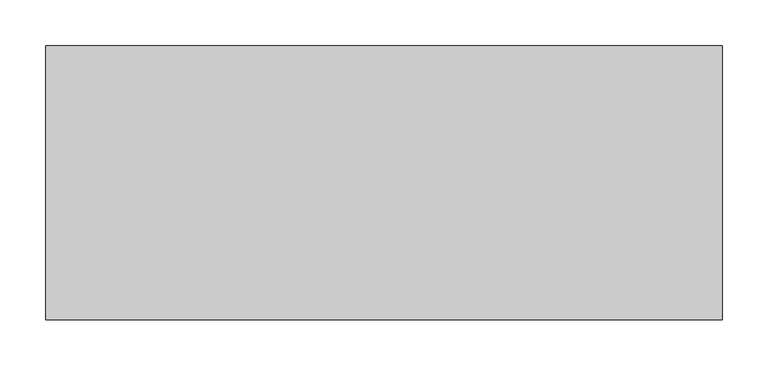
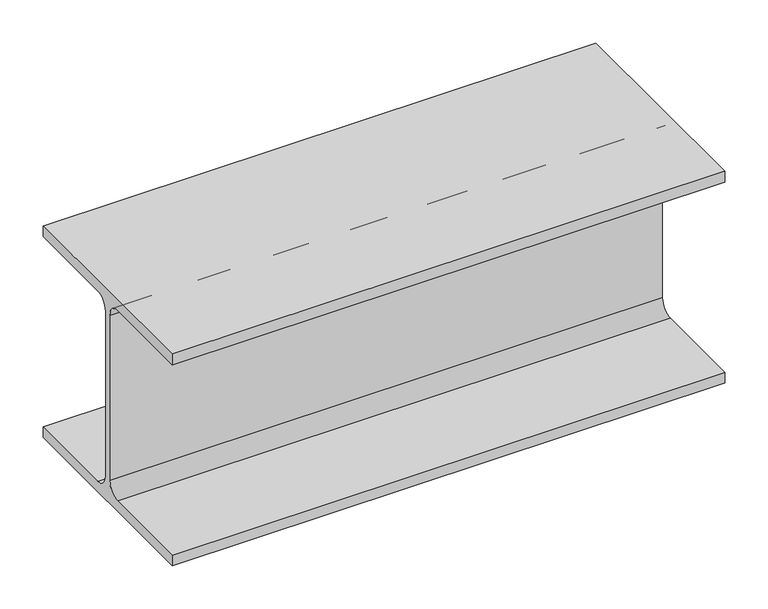
"""IFC4 building model written with IfcOpenShell, lengths in millimetres: beam geometry, 0912_Steel Framing_H-KSD3502 : H_SB_ASB_H-300x300x10x15."""

import ifcopenshell
import ifcopenshell.guid

model = None  # the IFC model being written
_history = None  # IfcOwnerHistory: only IFC2X3 demands one
_inside = {}  # id of a spatial element -> (the spatial element, [elements in it])
_under = {}  # id of a project, library or spatial element -> (it, [spatial elements below it])
_declared = {}  # id of a project -> (the project, [libraries it declares])
_typed = {}  # id of a type object -> (the type object, [elements of that type])
_made_of = {}  # id of a material, layer set ... -> (it, [elements and type objects made of it])


def new_model(schema):
    """Start an empty IFC model of exactly this schema.

    Asked for "IFC4X3", IfcOpenShell would pick the latest addendum, in which some entities
    have other attributes; the version numbers below select the first issue.
    IFC2X3 requires an IfcOwnerHistory on every rooted entity: one is made here for all.
    """
    global model, _history
    if schema == "IFC4X3":
        model = ifcopenshell.file(schema_version=(4, 3, 0, 0))
    else:
        model = ifcopenshell.file(schema=schema)
    _inside.clear()
    _under.clear()
    _declared.clear()
    _typed.clear()
    _made_of.clear()
    _history = None
    if model.schema == "IFC2X3":
        org = make("IfcOrganization", Name="unknown")
        user = make(
            "IfcPersonAndOrganization",
            ThePerson=make("IfcPerson", FamilyName="unknown"),
            TheOrganization=org,
        )
        app = make(
            "IfcApplication",
            ApplicationDeveloper=org,
            Version="unknown",
            ApplicationFullName="unknown",
            ApplicationIdentifier="unknown",
        )
        _history = make(
            "IfcOwnerHistory",
            OwningUser=user,
            OwningApplication=app,
            ChangeAction="ADDED",
            CreationDate=0,
        )
    return model


def make(cls, **values):
    """One entity of the class cls with the attributes given. An attribute that is None is left unset."""
    return model.create_entity(
        cls, **{name: value for name, value in values.items() if value is not None}
    )


def rooted(cls, **values):
    """An entity with a GlobalId (a new one), such as an element, a storey or a relation."""
    return make(cls, GlobalId=ifcopenshell.guid.new(), OwnerHistory=_history, **values)


def si_unit(unit_type, name, prefix=None):
    """IfcSIUnit, for example si_unit("LENGTHUNIT", "METRE", prefix="MILLI")."""
    return make("IfcSIUnit", UnitType=unit_type, Prefix=prefix, Name=name)


def assignment(units):
    """IfcUnitAssignment: the units of a project."""
    return None if units is None else make("IfcUnitAssignment", Units=units)


def point(xyz):
    """IfcCartesianPoint."""
    return None if xyz is None else make("IfcCartesianPoint", Coordinates=xyz)


def direction(xyz):
    """IfcDirection."""
    return None if xyz is None else make("IfcDirection", DirectionRatios=xyz)


def frame(location, z_axis=None, x_axis=None):
    """IfcAxis2Placement3D, a coordinate frame: its origin and axes. An axis left out is left unset."""
    return make(
        "IfcAxis2Placement3D",
        Location=point(location),
        Axis=direction(z_axis),
        RefDirection=direction(x_axis),
    )


def frame_2d(location, x_axis=None):
    """IfcAxis2Placement2D, a coordinate frame in the plane: its origin and x axis."""
    return make(
        "IfcAxis2Placement2D", Location=point(location), RefDirection=direction(x_axis)
    )


def origin():
    """The frame at (0, 0, 0) with its axes left unset."""
    return frame((0.0, 0.0, 0.0))


def place(relative_to, where):
    """IfcLocalPlacement: puts the frame where relative to a parent placement (None: the world)."""
    return make(
        "IfcLocalPlacement", PlacementRelTo=relative_to, RelativePlacement=where
    )


def context(
    kind, dimensions, precision=None, world=None, true_north=None, identifier=None
):
    """IfcGeometricRepresentationContext, for example the 3D "Model" context."""
    return make(
        "IfcGeometricRepresentationContext",
        ContextIdentifier=identifier,
        ContextType=kind,
        CoordinateSpaceDimension=dimensions,
        Precision=precision,
        WorldCoordinateSystem=world,
        TrueNorth=true_north,
    )


def project(units=None, contexts=None):
    """IfcProject with its units and contexts."""
    return rooted(
        "IfcProject",
        Name="project",
        RepresentationContexts=contexts,
        UnitsInContext=assignment(units),
    )


def spatial(cls, under=None, at=None, **own):
    """A site, building, storey or space (cls), placed at a placement, below another one or the project."""
    s = rooted(cls, ObjectPlacement=at, **own)
    if under is not None:
        _under.setdefault(under.id(), (under, []))[1].append(s)
    return s


def polyline(points):
    """IfcPolyline through the points."""
    return make("IfcPolyline", Points=[point(p) for p in points])


def circle_curve(where, radius):
    """IfcCircle in the frame where."""
    return make("IfcCircle", Position=where, Radius=radius)


def trimmed(basis, trim1, trim2, sense, master):
    """IfcTrimmedCurve: the piece of a basis curve between two trims."""
    return make(
        "IfcTrimmedCurve",
        BasisCurve=basis,
        Trim1=trim1,
        Trim2=trim2,
        SenseAgreement=sense,
        MasterRepresentation=master,
    )


def segment(curve, same_sense, transition):
    """IfcCompositeCurveSegment."""
    return make(
        "IfcCompositeCurveSegment",
        Transition=transition,
        SameSense=same_sense,
        ParentCurve=curve,
    )


def composite_curve(segments, self_intersect=None):
    """IfcCompositeCurve: segments joined end to end."""
    return make("IfcCompositeCurve", Segments=segments, SelfIntersect=self_intersect)


def outline(outer, holes=None, kind="AREA"):
    """IfcArbitraryClosedProfileDef: a profile drawn as a closed curve; with holes, ...WithVoids."""
    if holes is None:
        return make("IfcArbitraryClosedProfileDef", ProfileType=kind, OuterCurve=outer)
    return make(
        "IfcArbitraryProfileDefWithVoids",
        ProfileType=kind,
        OuterCurve=outer,
        InnerCurves=holes,
    )


def extrude(swept, where, along, depth):
    """IfcExtrudedAreaSolid: the profile swept, set in the frame where, extruded along a direction by depth."""
    return make(
        "IfcExtrudedAreaSolid",
        SweptArea=swept,
        Position=where,
        ExtrudedDirection=direction(along),
        Depth=depth,
    )


def shape(context_of_items, identifier, shape_type, items):
    """IfcShapeRepresentation: the items that make up one representation, for example the "Body"."""
    return make(
        "IfcShapeRepresentation",
        ContextOfItems=context_of_items,
        RepresentationIdentifier=identifier,
        RepresentationType=shape_type,
        Items=items,
    )


def source(mapping_origin, context_of_items, identifier, shape_type, items):
    """IfcRepresentationMap: a shape defined once, which mapped items show again and again."""
    return make(
        "IfcRepresentationMap",
        MappingOrigin=mapping_origin,
        MappedRepresentation=shape(context_of_items, identifier, shape_type, items),
    )


def transform(
    local_origin,
    x_axis=None,
    y_axis=None,
    z_axis=None,
    scale=None,
    scale2=None,
    scale3=None,
    uniform=True,
):
    """IfcCartesianTransformationOperator3D, or its non-uniform kind. x_axis, y_axis, z_axis: its Axis1, 2, 3."""
    if uniform:
        return make(
            "IfcCartesianTransformationOperator3D",
            Axis1=direction(x_axis),
            Axis2=direction(y_axis),
            LocalOrigin=point(local_origin),
            Scale=scale,
            Axis3=direction(z_axis),
        )
    return make(
        "IfcCartesianTransformationOperator3DnonUniform",
        Axis1=direction(x_axis),
        Axis2=direction(y_axis),
        LocalOrigin=point(local_origin),
        Scale=scale,
        Axis3=direction(z_axis),
        Scale2=scale2,
        Scale3=scale3,
    )


def mapped(mapping_source, mapping_target):
    """IfcMappedItem: shows the shape of a source again, moved by a transform."""
    return make(
        "IfcMappedItem", MappingSource=mapping_source, MappingTarget=mapping_target
    )


def made_of(thing, what):
    """Note that an element or type object is made of a material, layer set ...; save() writes the relation."""
    if what is not None:
        _made_of.setdefault(what.id(), (what, []))[1].append(thing)
    return thing


def element(
    cls,
    number,
    at=None,
    inside=None,
    cuts=None,
    type_object=None,
    material=None,
    context=None,
    identifier="Body",
    shape_type=None,
    held_by="IfcProductDefinitionShape",
    body=None,
    shapes=None,
    **own,
):
    """One element of the class cls, such as IfcWall. Its Tag is "e" and its number.

    at: its placement. inside: the storey or other place that contains it. cuts: it is an
    opening in that element (IfcRelVoidsElement). A single representation is given by context,
    identifier, shape_type and body (its items); several are given by shapes. held_by: the class
    of the entity that holds the representations. save() writes the other relations.
    """
    e = rooted(cls, Tag="e%d" % number, ObjectPlacement=at, **own)
    if body is not None:
        shapes = [shape(context, identifier, shape_type, body)]
    if shapes is not None:
        e.Representation = make(held_by, Representations=shapes)
    if inside is not None:
        _inside.setdefault(inside.id(), (inside, []))[1].append(e)
    if cuts is not None:
        rooted(
            "IfcRelVoidsElement", RelatingBuildingElement=cuts, RelatedOpeningElement=e
        )
    if type_object is not None:
        _typed.setdefault(type_object.id(), (type_object, []))[1].append(e)
    return made_of(e, material)


def aggregate(whole, parts):
    """IfcRelAggregates: a whole, such as a stair, and the parts it consists of."""
    return rooted("IfcRelAggregates", RelatingObject=whole, RelatedObjects=parts)


def save(model, path):
    """Write the relations noted so far, then the file.

    IfcRelAggregates (storeys below a building ...), IfcRelContainedInSpatialStructure (elements
    in a storey), IfcRelDefinesByType, IfcRelAssociatesMaterial and IfcRelDeclares: one each for
    every whole, place, type object, material and project.
    """
    for whole, parts in _under.values():
        aggregate(whole, parts)
    for where, things in _inside.values():
        rooted(
            "IfcRelContainedInSpatialStructure",
            RelatedElements=things,
            RelatingStructure=where,
        )
    for kind, things in _typed.values():
        rooted("IfcRelDefinesByType", RelatedObjects=things, RelatingType=kind)
    for what, things in _made_of.values():
        rooted("IfcRelAssociatesMaterial", RelatedObjects=things, RelatingMaterial=what)
    for by, libraries in _declared.values():
        rooted("IfcRelDeclares", RelatingContext=by, RelatedDefinitions=libraries)
    model.write(path)


def beam_a46f469d(model_context):
    return source(origin(), model_context, "Body", "SweptSolid", [
        extrude(outline(composite_curve([segment(polyline([(150.0, -135.0), (150.0, -150.0), (-150.0, -150.0), (-150.0, -135.0), (-23.0, -135.0)]), True, "CONTINUOUS"), segment(trimmed(circle_curve(frame_2d((-23.0, -117.0)), 18.0), [point((-23.0, -135.0))], [point((-5.0, -117.0))], True, "CARTESIAN"), True, "CONTINUOUS"), segment(polyline([(-5.0, -117.0), (-5.0, 117.0)]), True, "CONTINUOUS"), segment(trimmed(circle_curve(frame_2d((-23.0, 117.0)), 18.0), [point((-5.0, 117.0))], [point((-23.0, 135.0))], True, "CARTESIAN"), True, "CONTINUOUS"), segment(polyline([(-23.0, 135.0), (-150.0, 135.0), (-150.0, 150.0), (150.0, 150.0), (150.0, 135.0), (23.0, 135.0)]), True, "CONTINUOUS"), segment(trimmed(circle_curve(frame_2d((23.0, 117.0)), 18.0), [point((23.0, 135.0))], [point((5.0, 117.0))], True, "CARTESIAN"), True, "CONTINUOUS"), segment(polyline([(5.0, 117.0), (5.0, -117.0)]), True, "CONTINUOUS"), segment(trimmed(circle_curve(frame_2d((23.0, -117.0)), 18.0), [point((5.0, -117.0))], [point((23.0, -135.0))], True, "CARTESIAN"), True, "CONTINUOUS"), segment(polyline([(23.0, -135.0), (150.0, -135.0)]), True, "CONTINUOUS")], self_intersect=False)), frame((-502.4937811, 0.0, 0.0), z_axis=(1.0, 0.0, 0.0), x_axis=(0.0, 1.0, 0.0)), (0.0, 0.0, 1.0), 740.4687108),
    ])


if __name__ == "__main__":
    model = new_model("IFC4")
    model_context = context("Model", 3, world=origin())
    ifc_project = project(units=[si_unit("LENGTHUNIT", "METRE", prefix="MILLI")], contexts=[model_context])
    site = spatial("IfcSite", under=ifc_project)
    building = spatial("IfcBuilding", under=site)
    placement = place(None, origin())
    beam_shape = beam_a46f469d(model_context)
    element("IfcBeam", 1, ObjectType="0912_Steel Framing_H-KSD3502 : H_SB_ASB_H-300x300x10x15", at=placement, inside=building, context=model_context, shape_type="MappedRepresentation", body=[
        mapped(beam_shape, transform((0.0, 0.0, 0.0), x_axis=(1.0, 0.0, 0.0), y_axis=(0.0, 1.0, 0.0), z_axis=(0.0, 0.0, 1.0))),
    ])
    save(model, "model.ifc")

# Revit data of these elements
# Type "0912_Steel Framing_H-KSD3502 : H_SB_ASB_H-300x300x10x15"
#   H_WM Code_1 = "S01AA001-00001 | Main Steel Structure Fabrication Work | Shelter/Building | Heavy Steel - Standard (Weight≥90KG/M) | Material: (   )"
#   H_WM Code_2 = "S03AA027-00001 | Main Steel Structure Erection Work | Shelter/Building | Heavy Steel (Weight≥90KG/M) | Material: (   )"
#   H_WM Code_3 = "S01AA010-00001 | Main Steel Structure Fabrication Work | Shelter/Building | Steel Painting/Coating | for Non-Fireproofed Steel Surface, Surface Preparation, Primer, Second & Final Coat | Material: (   )"
#   H_Q'ty Cal Type Tag = "SB-Q2"
#   Width = 30.0 cm
#   Web Thickness = 1.0 cm
#   Web Fillet = 1.8 cm
#   Warping Constant = 1370000.0 cm⁶
#   W = 0
#   Torsional Moment of Inertia = 77.00 cm⁴
#   Section Area = 119.8 cm²
#   Plastic Modulus weak axis = 684.0 cm³
#   Plastic Modulus strong axis = 1500.0 cm³
#   Perimeter = 1.75 m²/m
#   Nominal Weight = 94.00 kgf/m
#   Moment of Inertia weak axis = 6750.00 cm⁴
#   Moment of Inertia strong axis = 20400.00 cm⁴
#   Height = 30.0 cm
#   Flange Thickness = 1.5 cm
#   Elastic Modulus weak axis = 450.0 cm³
#   Elastic Modulus strong axis = 1360.0 cm³
#   Centroid Vertical = 15.0 cm
#   Centroid Horizontal = 15.0 cm
#   Ix = 204000000
#   Length [instance default] = 1.5240 m
#   Zx = 1500000
#   b = 0.3000 m
#   h = 0.3000 m
#   r = 0.0180 m
#   s = 0.0100 m
#   t = 0.0150 m
#   A = 0.01198 m²
#   Structural Material [instance default] = Steel, 45-345
#   Assembly Code = ""
# Element 1 (IfcBeam, "0912_Steel Framing_H-KSD3502 : H_SB_ASB_H-300x300x10x15")
#   Structural Material = none
# Materials
#   "Steel, 45-345": class "Metal", colour RGB 189 187 185, transparency 0, Description = "Steel 345 MPa", Cost = 0
